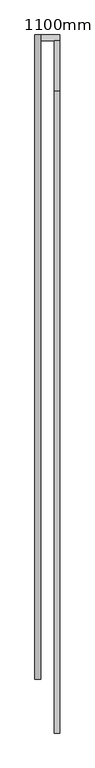
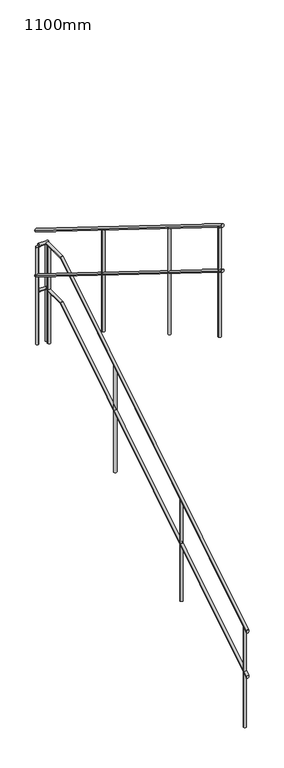
"""IFC4 building model written with IfcOpenShell, lengths in millimetres: railing geometry, 1100mm."""

import ifcopenshell
import ifcopenshell.guid

model = None  # the IFC model being written
_history = None  # IfcOwnerHistory: only IFC2X3 demands one
_inside = {}  # id of a spatial element -> (the spatial element, [elements in it])
_under = {}  # id of a project, library or spatial element -> (it, [spatial elements below it])
_declared = {}  # id of a project -> (the project, [libraries it declares])
_typed = {}  # id of a type object -> (the type object, [elements of that type])
_made_of = {}  # id of a material, layer set ... -> (it, [elements and type objects made of it])


def new_model(schema):
    """Start an empty IFC model of exactly this schema.

    Asked for "IFC4X3", IfcOpenShell would pick the latest addendum, in which some entities
    have other attributes; the version numbers below select the first issue.
    IFC2X3 requires an IfcOwnerHistory on every rooted entity: one is made here for all.
    """
    global model, _history
    if schema == "IFC4X3":
        model = ifcopenshell.file(schema_version=(4, 3, 0, 0))
    else:
        model = ifcopenshell.file(schema=schema)
    _inside.clear()
    _under.clear()
    _declared.clear()
    _typed.clear()
    _made_of.clear()
    _history = None
    if model.schema == "IFC2X3":
        org = make("IfcOrganization", Name="unknown")
        user = make(
            "IfcPersonAndOrganization",
            ThePerson=make("IfcPerson", FamilyName="unknown"),
            TheOrganization=org,
        )
        app = make(
            "IfcApplication",
            ApplicationDeveloper=org,
            Version="unknown",
            ApplicationFullName="unknown",
            ApplicationIdentifier="unknown",
        )
        _history = make(
            "IfcOwnerHistory",
            OwningUser=user,
            OwningApplication=app,
            ChangeAction="ADDED",
            CreationDate=0,
        )
    return model


def make(cls, **values):
    """One entity of the class cls with the attributes given. An attribute that is None is left unset."""
    return model.create_entity(
        cls, **{name: value for name, value in values.items() if value is not None}
    )


def rooted(cls, **values):
    """An entity with a GlobalId (a new one), such as an element, a storey or a relation."""
    return make(cls, GlobalId=ifcopenshell.guid.new(), OwnerHistory=_history, **values)


def si_unit(unit_type, name, prefix=None):
    """IfcSIUnit, for example si_unit("LENGTHUNIT", "METRE", prefix="MILLI")."""
    return make("IfcSIUnit", UnitType=unit_type, Prefix=prefix, Name=name)


def assignment(units):
    """IfcUnitAssignment: the units of a project."""
    return None if units is None else make("IfcUnitAssignment", Units=units)


def point(xyz):
    """IfcCartesianPoint."""
    return None if xyz is None else make("IfcCartesianPoint", Coordinates=xyz)


def direction(xyz):
    """IfcDirection."""
    return None if xyz is None else make("IfcDirection", DirectionRatios=xyz)


def frame(location, z_axis=None, x_axis=None):
    """IfcAxis2Placement3D, a coordinate frame: its origin and axes. An axis left out is left unset."""
    return make(
        "IfcAxis2Placement3D",
        Location=point(location),
        Axis=direction(z_axis),
        RefDirection=direction(x_axis),
    )


def frame_2d(location, x_axis=None):
    """IfcAxis2Placement2D, a coordinate frame in the plane: its origin and x axis."""
    return make(
        "IfcAxis2Placement2D", Location=point(location), RefDirection=direction(x_axis)
    )


def origin():
    """The frame at (0, 0, 0) with its axes left unset."""
    return frame((0.0, 0.0, 0.0))


def place(relative_to, where):
    """IfcLocalPlacement: puts the frame where relative to a parent placement (None: the world)."""
    return make(
        "IfcLocalPlacement", PlacementRelTo=relative_to, RelativePlacement=where
    )


def context(
    kind, dimensions, precision=None, world=None, true_north=None, identifier=None
):
    """IfcGeometricRepresentationContext, for example the 3D "Model" context."""
    return make(
        "IfcGeometricRepresentationContext",
        ContextIdentifier=identifier,
        ContextType=kind,
        CoordinateSpaceDimension=dimensions,
        Precision=precision,
        WorldCoordinateSystem=world,
        TrueNorth=true_north,
    )


def project(units=None, contexts=None):
    """IfcProject with its units and contexts."""
    return rooted(
        "IfcProject",
        Name="project",
        RepresentationContexts=contexts,
        UnitsInContext=assignment(units),
    )


def spatial(cls, under=None, at=None, **own):
    """A site, building, storey or space (cls), placed at a placement, below another one or the project."""
    s = rooted(cls, ObjectPlacement=at, **own)
    if under is not None:
        _under.setdefault(under.id(), (under, []))[1].append(s)
    return s


def circle_curve(where, radius):
    """IfcCircle in the frame where."""
    return make("IfcCircle", Position=where, Radius=radius)


def ellipse_curve(where, semi_axis1, semi_axis2):
    """IfcEllipse in the frame where."""
    return make(
        "IfcEllipse", Position=where, SemiAxis1=semi_axis1, SemiAxis2=semi_axis2
    )


def trimmed(basis, trim1, trim2, sense, master):
    """IfcTrimmedCurve: the piece of a basis curve between two trims."""
    return make(
        "IfcTrimmedCurve",
        BasisCurve=basis,
        Trim1=trim1,
        Trim2=trim2,
        SenseAgreement=sense,
        MasterRepresentation=master,
    )


def segment(curve, same_sense, transition):
    """IfcCompositeCurveSegment."""
    return make(
        "IfcCompositeCurveSegment",
        Transition=transition,
        SameSense=same_sense,
        ParentCurve=curve,
    )


def composite_curve(segments, self_intersect=None):
    """IfcCompositeCurve: segments joined end to end."""
    return make("IfcCompositeCurve", Segments=segments, SelfIntersect=self_intersect)


def outline(outer, holes=None, kind="AREA"):
    """IfcArbitraryClosedProfileDef: a profile drawn as a closed curve; with holes, ...WithVoids."""
    if holes is None:
        return make("IfcArbitraryClosedProfileDef", ProfileType=kind, OuterCurve=outer)
    return make(
        "IfcArbitraryProfileDefWithVoids",
        ProfileType=kind,
        OuterCurve=outer,
        InnerCurves=holes,
    )


def extrude(swept, where, along, depth):
    """IfcExtrudedAreaSolid: the profile swept, set in the frame where, extruded along a direction by depth."""
    return make(
        "IfcExtrudedAreaSolid",
        SweptArea=swept,
        Position=where,
        ExtrudedDirection=direction(along),
        Depth=depth,
    )


def shape(context_of_items, identifier, shape_type, items):
    """IfcShapeRepresentation: the items that make up one representation, for example the "Body"."""
    return make(
        "IfcShapeRepresentation",
        ContextOfItems=context_of_items,
        RepresentationIdentifier=identifier,
        RepresentationType=shape_type,
        Items=items,
    )


def source(mapping_origin, context_of_items, identifier, shape_type, items):
    """IfcRepresentationMap: a shape defined once, which mapped items show again and again."""
    return make(
        "IfcRepresentationMap",
        MappingOrigin=mapping_origin,
        MappedRepresentation=shape(context_of_items, identifier, shape_type, items),
    )


def transform(
    local_origin,
    x_axis=None,
    y_axis=None,
    z_axis=None,
    scale=None,
    scale2=None,
    scale3=None,
    uniform=True,
):
    """IfcCartesianTransformationOperator3D, or its non-uniform kind. x_axis, y_axis, z_axis: its Axis1, 2, 3."""
    if uniform:
        return make(
            "IfcCartesianTransformationOperator3D",
            Axis1=direction(x_axis),
            Axis2=direction(y_axis),
            LocalOrigin=point(local_origin),
            Scale=scale,
            Axis3=direction(z_axis),
        )
    return make(
        "IfcCartesianTransformationOperator3DnonUniform",
        Axis1=direction(x_axis),
        Axis2=direction(y_axis),
        LocalOrigin=point(local_origin),
        Scale=scale,
        Axis3=direction(z_axis),
        Scale2=scale2,
        Scale3=scale3,
    )


def mapped(mapping_source, mapping_target):
    """IfcMappedItem: shows the shape of a source again, moved by a transform."""
    return make(
        "IfcMappedItem", MappingSource=mapping_source, MappingTarget=mapping_target
    )


def made_of(thing, what):
    """Note that an element or type object is made of a material, layer set ...; save() writes the relation."""
    if what is not None:
        _made_of.setdefault(what.id(), (what, []))[1].append(thing)
    return thing


def element(
    cls,
    number,
    at=None,
    inside=None,
    cuts=None,
    type_object=None,
    material=None,
    context=None,
    identifier="Body",
    shape_type=None,
    held_by="IfcProductDefinitionShape",
    body=None,
    shapes=None,
    **own,
):
    """One element of the class cls, such as IfcWall. Its Tag is "e" and its number.

    at: its placement. inside: the storey or other place that contains it. cuts: it is an
    opening in that element (IfcRelVoidsElement). A single representation is given by context,
    identifier, shape_type and body (its items); several are given by shapes. held_by: the class
    of the entity that holds the representations. save() writes the other relations.
    """
    e = rooted(cls, Tag="e%d" % number, ObjectPlacement=at, **own)
    if body is not None:
        shapes = [shape(context, identifier, shape_type, body)]
    if shapes is not None:
        e.Representation = make(held_by, Representations=shapes)
    if inside is not None:
        _inside.setdefault(inside.id(), (inside, []))[1].append(e)
    if cuts is not None:
        rooted(
            "IfcRelVoidsElement", RelatingBuildingElement=cuts, RelatedOpeningElement=e
        )
    if type_object is not None:
        _typed.setdefault(type_object.id(), (type_object, []))[1].append(e)
    return made_of(e, material)


def aggregate(whole, parts):
    """IfcRelAggregates: a whole, such as a stair, and the parts it consists of."""
    return rooted("IfcRelAggregates", RelatingObject=whole, RelatedObjects=parts)


def save(model, path):
    """Write the relations noted so far, then the file.

    IfcRelAggregates (storeys below a building ...), IfcRelContainedInSpatialStructure (elements
    in a storey), IfcRelDefinesByType, IfcRelAssociatesMaterial and IfcRelDeclares: one each for
    every whole, place, type object, material and project.
    """
    for whole, parts in _under.values():
        aggregate(whole, parts)
    for where, things in _inside.values():
        rooted(
            "IfcRelContainedInSpatialStructure",
            RelatedElements=things,
            RelatingStructure=where,
        )
    for kind, things in _typed.values():
        rooted("IfcRelDefinesByType", RelatedObjects=things, RelatingType=kind)
    for what, things in _made_of.values():
        rooted("IfcRelAssociatesMaterial", RelatedObjects=things, RelatingMaterial=what)
    for by, libraries in _declared.values():
        rooted("IfcRelDeclares", RelatingContext=by, RelatedDefinitions=libraries)
    model.write(path)


def plane_surface(at):
    """IfcPlane: the flat surface through the origin of the frame at, square to its z axis."""
    return make("IfcPlane", Position=at)


def cylinder_surface(at, radius):
    """IfcCylindricalSurface: all points at the distance radius from the z axis of the frame at."""
    return make("IfcCylindricalSurface", Position=at, Radius=radius)


def advanced_brep(points, edges, surfaces, faces):
    """IfcAdvancedBrep: a solid bounded by faces that lie on surfaces and meet in shared edges.

    An edge is (start, end): straight between two places in points (the first is 0);
    or (start, end, curve); or (start, end, curve, False) where it runs against its curve.
    A face is (place in surfaces, loops), or (place, loops, False) where it looks against
    its surface's normal. A loop lists edges by number (the first is 1), with a minus sign
    where the edge is run from its end to its start. The first loop is the outer one.
    """
    corners = [point(p) for p in points]
    vertices = [make("IfcVertexPoint", VertexGeometry=c) for c in corners]
    made = []
    for start, end, *more in edges:
        made.append(
            make(
                "IfcEdgeCurve",
                EdgeStart=vertices[start],
                EdgeEnd=vertices[end],
                EdgeGeometry=more[0] if more else make("IfcPolyline", Points=[corners[start], corners[end]]),
                SameSense=more[1] if len(more) > 1 else True,
            )
        )
    hull = []
    for where, loops, *sense in faces:
        bounds = []
        for j, loop in enumerate(loops):
            ring = [make("IfcOrientedEdge", EdgeElement=made[abs(k) - 1], Orientation=k > 0) for k in loop]
            bounds.append(
                make(
                    "IfcFaceOuterBound" if j == 0 else "IfcFaceBound",
                    Bound=make("IfcEdgeLoop", EdgeList=ring),
                    Orientation=True,
                )
            )
        hull.append(make("IfcAdvancedFace", Bounds=bounds, FaceSurface=surfaces[where], SameSense=sense[0] if sense else True))
    return make("IfcAdvancedBrep", Outer=make("IfcClosedShell", CfsFaces=hull))


def railing_1100mm_37236d89(model_context):
    return source(origin(), model_context, "Body", "SolidModel", [
        advanced_brep(
        [(11540.5052251, 14699.5208589, 456.3396197), (11510.5052251, 14699.5208589, 456.3396197), (11540.5052251, 18324.9208589, 2547.0), (11510.5052251, 18324.9208589, 2547.0), (11540.5052251, 18063.8019306, 2547.0), (11510.5052251, 18063.8019306, 2547.0)],
        [
            (0, 1, ellipse_curve(frame((11525.5052251, 14699.5208589, 456.3396197), z_axis=(0.0, -1.0, 0.0), x_axis=(0.0, 0.0, -1.0)), 17.6603803, 15.0)),
            (1, 0, ellipse_curve(frame((11525.5052251, 14699.5208589, 456.3396197), z_axis=(0.0, -1.0, 0.0), x_axis=(0.0, 0.0, -1.0)), 17.6603803, 15.0)),
            (2, 3, circle_curve(frame((11525.5052251, 18324.9208589, 2547.0), z_axis=(0.0, 1.0, 0.0), x_axis=(-1.0, 0.0, 0.0)), 15.0)),
            (3, 2, circle_curve(frame((11525.5052251, 18324.9208589, 2547.0), z_axis=(0.0, 1.0, 0.0), x_axis=(-1.0, 0.0, 0.0)), 15.0)),
            (0, 4),
            (4, 5, ellipse_curve(frame((11525.5052251, 18063.8019306, 2547.0), z_axis=(0.0, -0.9616025257983003, -0.2744459552959912), x_axis=(0.0, 0.2744459552959914, -0.9616025257983002)), 15.5989607, 15.0)),
            (5, 1),
            (5, 4, ellipse_curve(frame((11525.5052251, 18063.8019306, 2547.0), z_axis=(0.0, -0.9616025257983003, -0.2744459552959912), x_axis=(0.0, 0.2744459552959914, -0.9616025257983002)), 15.5989607, 15.0)),
            (4, 2),
            (3, 5),
        ],
        [
            plane_surface(frame((11525.5052251, 14699.5208589, 474.0), z_axis=(0.0, -1.0, 0.0), x_axis=(0.0, 0.0, 1.0))),
            plane_surface(frame((11525.5052251, 18324.9208589, 2562.0), z_axis=(0.0, 1.0, 0.0), x_axis=(0.0, 0.0, 1.0))),
            cylinder_surface(frame((11525.5052251, 14707.4380966, 461.2596175), z_axis=(0.0, -0.8493588352433417, -0.5278158476155052), x_axis=(-1.0, 0.0, 0.0)), 15.0),
            cylinder_surface(frame((11525.5052251, 18059.5208589, 2547.0), z_axis=(0.0, -1.0, 0.0), x_axis=(-1.0, 0.0, 0.0)), 15.0),
        ],
        [
            (0, [[1, 2]]),
            (1, [[3, 4]]),
            (2, [[-1, 5, 6, 7]]),
            (2, [[-2, -7, 8, -5]]),
            (3, [[-6, 9, -4, 10]]),
            (3, [[-8, -10, -3, -9]]),
        ],
    ),
        advanced_brep(
        [(11540.5052251, 18354.9208589, 2547.0), (11540.5052251, 18324.9208589, 2547.0), (11439.7052251, 18354.9208589, 2547.0), (11439.7052251, 18324.9208589, 2547.0)],
        [
            (0, 1, circle_curve(frame((11540.5052251, 18339.9208589, 2547.0), z_axis=(1.0, 0.0, 0.0), x_axis=(0.0, -1.0, 0.0)), 15.0)),
            (1, 0, circle_curve(frame((11540.5052251, 18339.9208589, 2547.0), z_axis=(1.0, 0.0, 0.0), x_axis=(0.0, -1.0, 0.0)), 15.0)),
            (2, 3, circle_curve(frame((11439.7052251, 18339.9208589, 2547.0), z_axis=(-1.0, 0.0, 0.0), x_axis=(0.0, -1.0, 0.0)), 15.0)),
            (3, 2, circle_curve(frame((11439.7052251, 18339.9208589, 2547.0), z_axis=(-1.0, 0.0, 0.0), x_axis=(0.0, -1.0, 0.0)), 15.0)),
            (0, 2),
            (3, 1),
        ],
        [
            plane_surface(frame((11540.5052251, 18339.9208589, 2562.0), z_axis=(1.0, 0.0, 0.0), x_axis=(0.0, -1.0, 0.0))),
            plane_surface(frame((11439.7052251, 18339.9208589, 2562.0), z_axis=(-1.0, 0.0, 0.0), x_axis=(0.0, -1.0, 0.0))),
            cylinder_surface(frame((11540.5052251, 18339.9208589, 2547.0), z_axis=(1.0, 0.0, 0.0), x_axis=(0.0, -1.0, 0.0)), 15.0),
        ],
        [
            (0, [[1, 2]]),
            (1, [[3, 4]]),
            (2, [[-1, 5, -4, 6]]),
            (2, [[-2, -6, -3, -5]]),
        ],
    ),
        advanced_brep(
        [(11409.7052251, 18354.9208589, 2708.7696197), (11439.7052251, 18354.9208589, 2708.7696197), (11409.7052251, 14979.5208589, 4806.3396197), (11439.7052251, 14979.5208589, 4806.3396197)],
        [
            (0, 1, ellipse_curve(frame((11424.7052251, 18354.9208589, 2708.7696197), z_axis=(0.0, 1.0, 0.0), x_axis=(0.0, 0.0, -1.0)), 17.6603803, 15.0)),
            (1, 0, ellipse_curve(frame((11424.7052251, 18354.9208589, 2708.7696197), z_axis=(0.0, 1.0, 0.0), x_axis=(0.0, 0.0, -1.0)), 17.6603803, 15.0)),
            (2, 3, ellipse_curve(frame((11424.7052251, 14979.5208589, 4806.3396197), z_axis=(0.0, -1.0, 0.0), x_axis=(0.0, 0.0, -1.0)), 17.6603803, 15.0)),
            (3, 2, ellipse_curve(frame((11424.7052251, 14979.5208589, 4806.3396197), z_axis=(0.0, -1.0, 0.0), x_axis=(0.0, 0.0, -1.0)), 17.6603803, 15.0)),
            (0, 2),
            (3, 1),
        ],
        [
            plane_surface(frame((11424.7052251, 18354.9208589, 2726.43), z_axis=(0.0, 1.0, 0.0), x_axis=(0.0, 0.0, -1.0))),
            plane_surface(frame((11424.7052251, 14979.5208589, 4824.0), z_axis=(0.0, -1.0, 0.0), x_axis=(0.0, 0.0, -1.0))),
            cylinder_surface(frame((11424.7052251, 18347.0036212, 2713.6896175), z_axis=(0.0, 0.8493588352433417, -0.5278158476155052), x_axis=(1.0, 0.0, 0.0)), 15.0),
        ],
        [
            (0, [[1, 2]]),
            (1, [[3, 4]]),
            (2, [[-1, 5, -4, 6]]),
            (2, [[-2, -6, -3, -5]]),
        ],
    ),
        advanced_brep(
        [(11540.5052251, 14699.5208589, 956.3396197), (11510.5052251, 14699.5208589, 956.3396197), (11540.5052251, 18063.8019306, 3047.0), (11510.5052251, 18063.8019306, 3047.0), (11540.5052251, 18324.9208589, 3047.0), (11510.5052251, 18324.9208589, 3047.0)],
        [
            (0, 1, ellipse_curve(frame((11525.5052251, 14699.5208589, 956.3396197), z_axis=(0.0, -1.0, 0.0), x_axis=(0.0, 0.0, -1.0)), 17.6603803, 15.0)),
            (1, 0, ellipse_curve(frame((11525.5052251, 14699.5208589, 956.3396197), z_axis=(0.0, -1.0, 0.0), x_axis=(0.0, 0.0, -1.0)), 17.6603803, 15.0)),
            (0, 2),
            (2, 3, ellipse_curve(frame((11525.5052251, 18063.8019306, 3047.0), z_axis=(0.0, -0.9616025257983003, -0.2744459552959912), x_axis=(0.0, 0.2744459552959914, -0.9616025257983002)), 15.5989607, 15.0)),
            (3, 1),
            (3, 2, ellipse_curve(frame((11525.5052251, 18063.8019306, 3047.0), z_axis=(0.0, -0.9616025257983003, -0.2744459552959912), x_axis=(0.0, 0.2744459552959914, -0.9616025257983002)), 15.5989607, 15.0)),
            (4, 5, circle_curve(frame((11525.5052251, 18324.9208589, 3047.0), z_axis=(0.0, 1.0, 0.0), x_axis=(-1.0, 0.0, 0.0)), 15.0)),
            (5, 4, circle_curve(frame((11525.5052251, 18324.9208589, 3047.0), z_axis=(0.0, 1.0, 0.0), x_axis=(-1.0, 0.0, 0.0)), 15.0)),
            (2, 4),
            (5, 3),
        ],
        [
            plane_surface(frame((11525.5052251, 14699.5208589, 974.0), z_axis=(0.0, -1.0, 0.0), x_axis=(0.0, 0.0, 1.0))),
            cylinder_surface(frame((11525.5052251, 14707.4380966, 961.2596175), z_axis=(0.0, -0.8493588352433417, -0.5278158476155052), x_axis=(-1.0, 0.0, 0.0)), 15.0),
            plane_surface(frame((11525.5052251, 18324.9208589, 3062.0), z_axis=(0.0, 1.0, 0.0), x_axis=(0.0, 0.0, 1.0))),
            cylinder_surface(frame((11525.5052251, 18059.5208589, 3047.0), z_axis=(0.0, -1.0, 0.0), x_axis=(-1.0, 0.0, 0.0)), 15.0),
        ],
        [
            (0, [[1, 2]]),
            (1, [[-1, 3, 4, 5]]),
            (1, [[-2, -5, 6, -3]]),
            (2, [[7, 8]]),
            (3, [[-4, 9, -8, 10]]),
            (3, [[-6, -10, -7, -9]]),
        ],
    ),
        advanced_brep(
        [(11540.5052251, 18354.9208589, 3047.0), (11540.5052251, 18324.9208589, 3047.0), (11439.7052251, 18354.9208589, 3047.0), (11439.7052251, 18324.9208589, 3047.0)],
        [
            (0, 1, circle_curve(frame((11540.5052251, 18339.9208589, 3047.0), z_axis=(1.0, 0.0, 0.0), x_axis=(0.0, -1.0, 0.0)), 15.0)),
            (1, 0, circle_curve(frame((11540.5052251, 18339.9208589, 3047.0), z_axis=(1.0, 0.0, 0.0), x_axis=(0.0, -1.0, 0.0)), 15.0)),
            (2, 3, circle_curve(frame((11439.7052251, 18339.9208589, 3047.0), z_axis=(-1.0, 0.0, 0.0), x_axis=(0.0, -1.0, 0.0)), 15.0)),
            (3, 2, circle_curve(frame((11439.7052251, 18339.9208589, 3047.0), z_axis=(-1.0, 0.0, 0.0), x_axis=(0.0, -1.0, 0.0)), 15.0)),
            (0, 2),
            (3, 1),
        ],
        [
            plane_surface(frame((11540.5052251, 18339.9208589, 3062.0), z_axis=(1.0, 0.0, 0.0), x_axis=(0.0, -1.0, 0.0))),
            plane_surface(frame((11439.7052251, 18339.9208589, 3062.0), z_axis=(-1.0, 0.0, 0.0), x_axis=(0.0, -1.0, 0.0))),
            cylinder_surface(frame((11540.5052251, 18339.9208589, 3047.0), z_axis=(1.0, 0.0, 0.0), x_axis=(0.0, -1.0, 0.0)), 15.0),
        ],
        [
            (0, [[1, 2]]),
            (1, [[3, 4]]),
            (2, [[-1, 5, -4, 6]]),
            (2, [[-2, -6, -3, -5]]),
        ],
    ),
        advanced_brep(
        [(11409.7052251, 18354.9208589, 3208.7696197), (11439.7052251, 18354.9208589, 3208.7696197), (11409.7052251, 14979.5208589, 5306.3396197), (11439.7052251, 14979.5208589, 5306.3396197)],
        [
            (0, 1, ellipse_curve(frame((11424.7052251, 18354.9208589, 3208.7696197), z_axis=(0.0, 1.0, 0.0), x_axis=(0.0, 0.0, -1.0)), 17.6603803, 15.0)),
            (1, 0, ellipse_curve(frame((11424.7052251, 18354.9208589, 3208.7696197), z_axis=(0.0, 1.0, 0.0), x_axis=(0.0, 0.0, -1.0)), 17.6603803, 15.0)),
            (2, 3, ellipse_curve(frame((11424.7052251, 14979.5208589, 5306.3396197), z_axis=(0.0, -1.0, 0.0), x_axis=(0.0, 0.0, -1.0)), 17.6603803, 15.0)),
            (3, 2, ellipse_curve(frame((11424.7052251, 14979.5208589, 5306.3396197), z_axis=(0.0, -1.0, 0.0), x_axis=(0.0, 0.0, -1.0)), 17.6603803, 15.0)),
            (0, 2),
            (3, 1),
        ],
        [
            plane_surface(frame((11424.7052251, 18354.9208589, 3226.43), z_axis=(0.0, 1.0, 0.0), x_axis=(0.0, 0.0, -1.0))),
            plane_surface(frame((11424.7052251, 14979.5208589, 5324.0), z_axis=(0.0, -1.0, 0.0), x_axis=(0.0, 0.0, -1.0))),
            cylinder_surface(frame((11424.7052251, 18347.0036212, 3213.6896175), z_axis=(0.0, 0.8493588352433417, -0.5278158476155052), x_axis=(1.0, 0.0, 0.0)), 15.0),
        ],
        [
            (0, [[1, 2]]),
            (1, [[3, 4]]),
            (2, [[-1, 5, -4, 6]]),
            (2, [[-2, -6, -3, -5]]),
        ],
    ),
        extrude(outline(composite_curve([segment(trimmed(circle_curve(frame_2d((11424.7052251, 15939.9208589)), 15.0), [point((11439.7052251, 15939.9208589))], [point((11409.7052251, 15939.9208589))], False, "CARTESIAN"), True, "CONTINUOUS"), segment(trimmed(circle_curve(frame_2d((11424.7052251, 15939.9208589)), 15.0), [point((11409.7052251, 15939.9208589))], [point((11439.7052251, 15939.9208589))], False, "CARTESIAN"), True, "CONTINUOUS")], self_intersect=False)), frame((0.0, 0.0, 3528.0), z_axis=(0.0, 0.0, 1.0), x_axis=(1.0, 0.0, 0.0)), (0.0, 0.0, 1.0), 1169.18),
        extrude(outline(composite_curve([segment(trimmed(circle_curve(frame_2d((11424.7052251, 17139.9208589)), 15.0), [point((11439.7052251, 17139.9208589))], [point((11409.7052251, 17139.9208589))], False, "CARTESIAN"), True, "CONTINUOUS"), segment(trimmed(circle_curve(frame_2d((11424.7052251, 17139.9208589)), 15.0), [point((11409.7052251, 17139.9208589))], [point((11439.7052251, 17139.9208589))], False, "CARTESIAN"), True, "CONTINUOUS")], self_intersect=False)), frame((0.0, 0.0, 2832.0), z_axis=(0.0, 0.0, 1.0), x_axis=(1.0, 0.0, 0.0)), (0.0, 0.0, 1.0), 1119.4657143),
        extrude(outline(composite_curve([segment(trimmed(circle_curve(frame_2d((11525.5052251, 18299.5208589)), 15.0), [point((11510.5052251, 18299.5208589))], [point((11540.5052251, 18299.5208589))], False, "CARTESIAN"), True, "CONTINUOUS"), segment(trimmed(circle_curve(frame_2d((11525.5052251, 18299.5208589)), 15.0), [point((11540.5052251, 18299.5208589))], [point((11510.5052251, 18299.5208589))], False, "CARTESIAN"), True, "CONTINUOUS")], self_intersect=False)), frame((0.0, 0.0, 1962.0), z_axis=(0.0, 0.0, 1.0), x_axis=(1.0, 0.0, 0.0)), (0.0, 0.0, 1.0), 1070.0),
        extrude(outline(composite_curve([segment(trimmed(circle_curve(frame_2d((11525.5052251, 17099.5208589)), 15.0), [point((11510.5052251, 17099.5208589))], [point((11540.5052251, 17099.5208589))], False, "CARTESIAN"), True, "CONTINUOUS"), segment(trimmed(circle_curve(frame_2d((11525.5052251, 17099.5208589)), 15.0), [point((11540.5052251, 17099.5208589))], [point((11510.5052251, 17099.5208589))], False, "CARTESIAN"), True, "CONTINUOUS")], self_intersect=False)), frame((0.0, 0.0, 1266.0), z_axis=(0.0, 0.0, 1.0), x_axis=(1.0, 0.0, 0.0)), (0.0, 0.0, 1.0), 1169.4285714),
        extrude(outline(composite_curve([segment(trimmed(circle_curve(frame_2d((11525.5052251, 15899.5208589)), 15.0), [point((11510.5052251, 15899.5208589))], [point((11540.5052251, 15899.5208589))], False, "CARTESIAN"), True, "CONTINUOUS"), segment(trimmed(circle_curve(frame_2d((11525.5052251, 15899.5208589)), 15.0), [point((11540.5052251, 15899.5208589))], [point((11510.5052251, 15899.5208589))], False, "CARTESIAN"), True, "CONTINUOUS")], self_intersect=False)), frame((0.0, 0.0, 570.0), z_axis=(0.0, 0.0, 1.0), x_axis=(1.0, 0.0, 0.0)), (0.0, 0.0, 1.0), 1119.7142857),
        extrude(outline(composite_curve([segment(trimmed(circle_curve(frame_2d((11424.7052251, 18339.9208589)), 15.0), [point((11424.7052251, 18324.9208589))], [point((11424.7052251, 18354.9208589))], False, "CARTESIAN"), True, "CONTINUOUS"), segment(trimmed(circle_curve(frame_2d((11424.7052251, 18339.9208589)), 15.0), [point((11424.7052251, 18354.9208589))], [point((11424.7052251, 18324.9208589))], False, "CARTESIAN"), True, "CONTINUOUS")], self_intersect=False)), frame((0.0, 0.0, 1962.0), z_axis=(0.0, 0.0, 1.0), x_axis=(1.0, 0.0, 0.0)), (0.0, 0.0, 1.0), 1070.0),
        extrude(outline(composite_curve([segment(trimmed(circle_curve(frame_2d((11525.5052251, 18339.9208589)), 15.0), [point((11510.5052251, 18339.9208589))], [point((11540.5052251, 18339.9208589))], False, "CARTESIAN"), True, "CONTINUOUS"), segment(trimmed(circle_curve(frame_2d((11525.5052251, 18339.9208589)), 15.0), [point((11540.5052251, 18339.9208589))], [point((11510.5052251, 18339.9208589))], False, "CARTESIAN"), True, "CONTINUOUS")], self_intersect=False)), frame((0.0, 0.0, 1962.0), z_axis=(0.0, 0.0, 1.0), x_axis=(1.0, 0.0, 0.0)), (0.0, 0.0, 1.0), 1070.0),
        extrude(outline(composite_curve([segment(trimmed(circle_curve(frame_2d((11424.7052251, 15029.5208589)), 15.0), [point((11439.7052251, 15029.5208589))], [point((11409.7052251, 15029.5208589))], False, "CARTESIAN"), True, "CONTINUOUS"), segment(trimmed(circle_curve(frame_2d((11424.7052251, 15029.5208589)), 15.0), [point((11409.7052251, 15029.5208589))], [point((11439.7052251, 15029.5208589))], False, "CARTESIAN"), True, "CONTINUOUS")], self_intersect=False)), frame((0.0, 0.0, 4050.0), z_axis=(0.0, 0.0, 1.0), x_axis=(1.0, 0.0, 0.0)), (0.0, 0.0, 1.0), 1212.9285714),
        extrude(outline(composite_curve([segment(trimmed(circle_curve(frame_2d((11525.5052251, 14749.5208589)), 15.0), [point((11510.5052251, 14749.5208589))], [point((11540.5052251, 14749.5208589))], False, "CARTESIAN"), True, "CONTINUOUS"), segment(trimmed(circle_curve(frame_2d((11525.5052251, 14749.5208589)), 15.0), [point((11540.5052251, 14749.5208589))], [point((11510.5052251, 14749.5208589))], False, "CARTESIAN"), True, "CONTINUOUS")], self_intersect=False)), frame((0.0, 0.0, -126.0), z_axis=(0.0, 0.0, 1.0), x_axis=(1.0, 0.0, 0.0)), (0.0, 0.0, 1.0), 1101.0714286),
    ])


if __name__ == "__main__":
    model = new_model("IFC4")
    model_context = context("Model", 3, world=origin())
    ifc_project = project(units=[si_unit("LENGTHUNIT", "METRE", prefix="MILLI")], contexts=[model_context])
    site = spatial("IfcSite", under=ifc_project)
    building = spatial("IfcBuilding", under=site)
    placement = place(None, origin())
    railing_1100mm_shape = railing_1100mm_37236d89(model_context)
    element("IfcRailing", 1, ObjectType="1100mm", at=placement, inside=building, context=model_context, shape_type="MappedRepresentation", body=[
        mapped(railing_1100mm_shape, transform((0.0, 0.0, 0.0), x_axis=(1.0, 0.0, 0.0), y_axis=(0.0, 1.0, 0.0), z_axis=(0.0, 0.0, 1.0))),
    ])
    save(model, "model.ifc")
